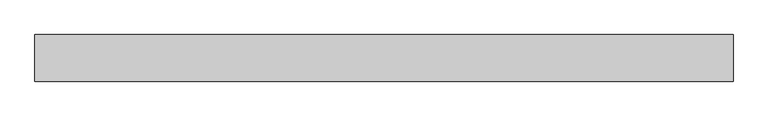
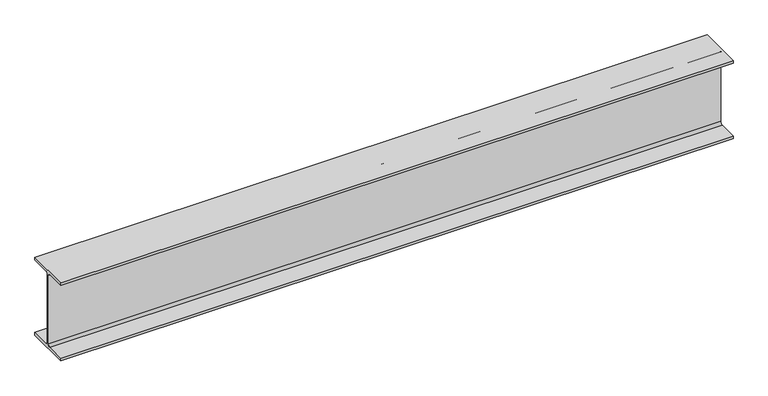
"""IFC4 building model written with IfcOpenShell, lengths in millimetres: beam geometry, Old_Steel Beam_H-KSD3502 : H_SB_ASB_H-350×175x7x11."""

import ifcopenshell
import ifcopenshell.guid

model = None  # the IFC model being written
_history = None  # IfcOwnerHistory: only IFC2X3 demands one
_inside = {}  # id of a spatial element -> (the spatial element, [elements in it])
_under = {}  # id of a project, library or spatial element -> (it, [spatial elements below it])
_declared = {}  # id of a project -> (the project, [libraries it declares])
_typed = {}  # id of a type object -> (the type object, [elements of that type])
_made_of = {}  # id of a material, layer set ... -> (it, [elements and type objects made of it])


def new_model(schema):
    """Start an empty IFC model of exactly this schema.

    Asked for "IFC4X3", IfcOpenShell would pick the latest addendum, in which some entities
    have other attributes; the version numbers below select the first issue.
    IFC2X3 requires an IfcOwnerHistory on every rooted entity: one is made here for all.
    """
    global model, _history
    if schema == "IFC4X3":
        model = ifcopenshell.file(schema_version=(4, 3, 0, 0))
    else:
        model = ifcopenshell.file(schema=schema)
    _inside.clear()
    _under.clear()
    _declared.clear()
    _typed.clear()
    _made_of.clear()
    _history = None
    if model.schema == "IFC2X3":
        org = make("IfcOrganization", Name="unknown")
        user = make(
            "IfcPersonAndOrganization",
            ThePerson=make("IfcPerson", FamilyName="unknown"),
            TheOrganization=org,
        )
        app = make(
            "IfcApplication",
            ApplicationDeveloper=org,
            Version="unknown",
            ApplicationFullName="unknown",
            ApplicationIdentifier="unknown",
        )
        _history = make(
            "IfcOwnerHistory",
            OwningUser=user,
            OwningApplication=app,
            ChangeAction="ADDED",
            CreationDate=0,
        )
    return model


def make(cls, **values):
    """One entity of the class cls with the attributes given. An attribute that is None is left unset."""
    return model.create_entity(
        cls, **{name: value for name, value in values.items() if value is not None}
    )


def rooted(cls, **values):
    """An entity with a GlobalId (a new one), such as an element, a storey or a relation."""
    return make(cls, GlobalId=ifcopenshell.guid.new(), OwnerHistory=_history, **values)


def si_unit(unit_type, name, prefix=None):
    """IfcSIUnit, for example si_unit("LENGTHUNIT", "METRE", prefix="MILLI")."""
    return make("IfcSIUnit", UnitType=unit_type, Prefix=prefix, Name=name)


def assignment(units):
    """IfcUnitAssignment: the units of a project."""
    return None if units is None else make("IfcUnitAssignment", Units=units)


def point(xyz):
    """IfcCartesianPoint."""
    return None if xyz is None else make("IfcCartesianPoint", Coordinates=xyz)


def direction(xyz):
    """IfcDirection."""
    return None if xyz is None else make("IfcDirection", DirectionRatios=xyz)


def frame(location, z_axis=None, x_axis=None):
    """IfcAxis2Placement3D, a coordinate frame: its origin and axes. An axis left out is left unset."""
    return make(
        "IfcAxis2Placement3D",
        Location=point(location),
        Axis=direction(z_axis),
        RefDirection=direction(x_axis),
    )


def frame_2d(location, x_axis=None):
    """IfcAxis2Placement2D, a coordinate frame in the plane: its origin and x axis."""
    return make(
        "IfcAxis2Placement2D", Location=point(location), RefDirection=direction(x_axis)
    )


def origin():
    """The frame at (0, 0, 0) with its axes left unset."""
    return frame((0.0, 0.0, 0.0))


def place(relative_to, where):
    """IfcLocalPlacement: puts the frame where relative to a parent placement (None: the world)."""
    return make(
        "IfcLocalPlacement", PlacementRelTo=relative_to, RelativePlacement=where
    )


def context(
    kind, dimensions, precision=None, world=None, true_north=None, identifier=None
):
    """IfcGeometricRepresentationContext, for example the 3D "Model" context."""
    return make(
        "IfcGeometricRepresentationContext",
        ContextIdentifier=identifier,
        ContextType=kind,
        CoordinateSpaceDimension=dimensions,
        Precision=precision,
        WorldCoordinateSystem=world,
        TrueNorth=true_north,
    )


def project(units=None, contexts=None):
    """IfcProject with its units and contexts."""
    return rooted(
        "IfcProject",
        Name="project",
        RepresentationContexts=contexts,
        UnitsInContext=assignment(units),
    )


def spatial(cls, under=None, at=None, **own):
    """A site, building, storey or space (cls), placed at a placement, below another one or the project."""
    s = rooted(cls, ObjectPlacement=at, **own)
    if under is not None:
        _under.setdefault(under.id(), (under, []))[1].append(s)
    return s


def polyline(points):
    """IfcPolyline through the points."""
    return make("IfcPolyline", Points=[point(p) for p in points])


def circle_curve(where, radius):
    """IfcCircle in the frame where."""
    return make("IfcCircle", Position=where, Radius=radius)


def trimmed(basis, trim1, trim2, sense, master):
    """IfcTrimmedCurve: the piece of a basis curve between two trims."""
    return make(
        "IfcTrimmedCurve",
        BasisCurve=basis,
        Trim1=trim1,
        Trim2=trim2,
        SenseAgreement=sense,
        MasterRepresentation=master,
    )


def segment(curve, same_sense, transition):
    """IfcCompositeCurveSegment."""
    return make(
        "IfcCompositeCurveSegment",
        Transition=transition,
        SameSense=same_sense,
        ParentCurve=curve,
    )


def composite_curve(segments, self_intersect=None):
    """IfcCompositeCurve: segments joined end to end."""
    return make("IfcCompositeCurve", Segments=segments, SelfIntersect=self_intersect)


def outline(outer, holes=None, kind="AREA"):
    """IfcArbitraryClosedProfileDef: a profile drawn as a closed curve; with holes, ...WithVoids."""
    if holes is None:
        return make("IfcArbitraryClosedProfileDef", ProfileType=kind, OuterCurve=outer)
    return make(
        "IfcArbitraryProfileDefWithVoids",
        ProfileType=kind,
        OuterCurve=outer,
        InnerCurves=holes,
    )


def extrude(swept, where, along, depth):
    """IfcExtrudedAreaSolid: the profile swept, set in the frame where, extruded along a direction by depth."""
    return make(
        "IfcExtrudedAreaSolid",
        SweptArea=swept,
        Position=where,
        ExtrudedDirection=direction(along),
        Depth=depth,
    )


def shape(context_of_items, identifier, shape_type, items):
    """IfcShapeRepresentation: the items that make up one representation, for example the "Body"."""
    return make(
        "IfcShapeRepresentation",
        ContextOfItems=context_of_items,
        RepresentationIdentifier=identifier,
        RepresentationType=shape_type,
        Items=items,
    )


def source(mapping_origin, context_of_items, identifier, shape_type, items):
    """IfcRepresentationMap: a shape defined once, which mapped items show again and again."""
    return make(
        "IfcRepresentationMap",
        MappingOrigin=mapping_origin,
        MappedRepresentation=shape(context_of_items, identifier, shape_type, items),
    )


def transform(
    local_origin,
    x_axis=None,
    y_axis=None,
    z_axis=None,
    scale=None,
    scale2=None,
    scale3=None,
    uniform=True,
):
    """IfcCartesianTransformationOperator3D, or its non-uniform kind. x_axis, y_axis, z_axis: its Axis1, 2, 3."""
    if uniform:
        return make(
            "IfcCartesianTransformationOperator3D",
            Axis1=direction(x_axis),
            Axis2=direction(y_axis),
            LocalOrigin=point(local_origin),
            Scale=scale,
            Axis3=direction(z_axis),
        )
    return make(
        "IfcCartesianTransformationOperator3DnonUniform",
        Axis1=direction(x_axis),
        Axis2=direction(y_axis),
        LocalOrigin=point(local_origin),
        Scale=scale,
        Axis3=direction(z_axis),
        Scale2=scale2,
        Scale3=scale3,
    )


def mapped(mapping_source, mapping_target):
    """IfcMappedItem: shows the shape of a source again, moved by a transform."""
    return make(
        "IfcMappedItem", MappingSource=mapping_source, MappingTarget=mapping_target
    )


def made_of(thing, what):
    """Note that an element or type object is made of a material, layer set ...; save() writes the relation."""
    if what is not None:
        _made_of.setdefault(what.id(), (what, []))[1].append(thing)
    return thing


def element(
    cls,
    number,
    at=None,
    inside=None,
    cuts=None,
    type_object=None,
    material=None,
    context=None,
    identifier="Body",
    shape_type=None,
    held_by="IfcProductDefinitionShape",
    body=None,
    shapes=None,
    **own,
):
    """One element of the class cls, such as IfcWall. Its Tag is "e" and its number.

    at: its placement. inside: the storey or other place that contains it. cuts: it is an
    opening in that element (IfcRelVoidsElement). A single representation is given by context,
    identifier, shape_type and body (its items); several are given by shapes. held_by: the class
    of the entity that holds the representations. save() writes the other relations.
    """
    e = rooted(cls, Tag="e%d" % number, ObjectPlacement=at, **own)
    if body is not None:
        shapes = [shape(context, identifier, shape_type, body)]
    if shapes is not None:
        e.Representation = make(held_by, Representations=shapes)
    if inside is not None:
        _inside.setdefault(inside.id(), (inside, []))[1].append(e)
    if cuts is not None:
        rooted(
            "IfcRelVoidsElement", RelatingBuildingElement=cuts, RelatedOpeningElement=e
        )
    if type_object is not None:
        _typed.setdefault(type_object.id(), (type_object, []))[1].append(e)
    return made_of(e, material)


def aggregate(whole, parts):
    """IfcRelAggregates: a whole, such as a stair, and the parts it consists of."""
    return rooted("IfcRelAggregates", RelatingObject=whole, RelatedObjects=parts)


def save(model, path):
    """Write the relations noted so far, then the file.

    IfcRelAggregates (storeys below a building ...), IfcRelContainedInSpatialStructure (elements
    in a storey), IfcRelDefinesByType, IfcRelAssociatesMaterial and IfcRelDeclares: one each for
    every whole, place, type object, material and project.
    """
    for whole, parts in _under.values():
        aggregate(whole, parts)
    for where, things in _inside.values():
        rooted(
            "IfcRelContainedInSpatialStructure",
            RelatedElements=things,
            RelatingStructure=where,
        )
    for kind, things in _typed.values():
        rooted("IfcRelDefinesByType", RelatedObjects=things, RelatingType=kind)
    for what, things in _made_of.values():
        rooted("IfcRelAssociatesMaterial", RelatedObjects=things, RelatingMaterial=what)
    for by, libraries in _declared.values():
        rooted("IfcRelDeclares", RelatingContext=by, RelatedDefinitions=libraries)
    model.write(path)


def beam_ab680fa0(model_context):
    return source(origin(), model_context, "Body", "SweptSolid", [
        extrude(outline(composite_curve([segment(polyline([(82.5, -141.5), (82.5, -151.7), (-82.5, -151.7), (-82.5, -141.5), (-11.9, -141.5)]), True, "CONTINUOUS"), segment(trimmed(circle_curve(frame_2d((-11.9, -132.6)), 8.9), [point((-11.9, -141.5))], [point((-3.0, -132.6))], True, "CARTESIAN"), True, "CONTINUOUS"), segment(polyline([(-3.0, -132.6), (-3.0, 132.6)]), True, "CONTINUOUS"), segment(trimmed(circle_curve(frame_2d((-11.9, 132.6)), 8.9), [point((-3.0, 132.6))], [point((-11.9, 141.5))], True, "CARTESIAN"), True, "CONTINUOUS"), segment(polyline([(-11.9, 141.5), (-82.5, 141.5), (-82.5, 151.7), (82.5, 151.7), (82.5, 141.5), (11.9, 141.5)]), True, "CONTINUOUS"), segment(trimmed(circle_curve(frame_2d((11.9, 132.6)), 8.9), [point((11.9, 141.5))], [point((3.0, 132.6))], True, "CARTESIAN"), True, "CONTINUOUS"), segment(polyline([(3.0, 132.6), (3.0, -132.6)]), True, "CONTINUOUS"), segment(trimmed(circle_curve(frame_2d((11.9, -132.6)), 8.9), [point((3.0, -132.6))], [point((11.9, -141.5))], True, "CARTESIAN"), True, "CONTINUOUS"), segment(polyline([(11.9, -141.5), (82.5, -141.5)]), True, "CONTINUOUS")], self_intersect=False)), frame((-1295.7739051, 0.0, 0.0), z_axis=(1.0, 0.0, 0.0), x_axis=(0.0, 1.0, 0.0)), (0.0, 0.0, 1.0), 2471.4118659),
    ])


if __name__ == "__main__":
    model = new_model("IFC4")
    model_context = context("Model", 3, world=origin())
    ifc_project = project(units=[si_unit("LENGTHUNIT", "METRE", prefix="MILLI")], contexts=[model_context])
    site = spatial("IfcSite", under=ifc_project)
    building = spatial("IfcBuilding", under=site)
    placement = place(None, origin())
    beam_shape = beam_ab680fa0(model_context)
    element("IfcBeam", 1, ObjectType="Old_Steel Beam_H-KSD3502 : H_SB_ASB_H-350×175x7x11", at=placement, inside=building, context=model_context, shape_type="MappedRepresentation", body=[
        mapped(beam_shape, transform((0.0, 0.0, 0.0), x_axis=(1.0, 0.0, 0.0), y_axis=(0.0, 1.0, 0.0), z_axis=(0.0, 0.0, 1.0))),
    ])
    save(model, "model.ifc")

# Revit data of these elements
# Type "Old_Steel Beam_H-KSD3502 : H_SB_ASB_H-350×175x7x11"
#   Width = 17.5 cm
#   Web Thickness = 0.7 cm
#   Web Fillet = 1.4 cm
#   Warping Constant = 282290.0 cm⁶
#   Torsional Moment of Inertia = 19.4042 cm⁴
#   Torsional Modulus = 1.0 cm³
#   Section Area = 63.14 cm²
#   Plastic Modulus weak axis = 174.0 cm³
#   Plastic Modulus strong axis = 868.0 cm³
#   Perimeter = 1.36 m²/m
#   Nominal Weight = 49.60 kgf/m
#   Moment of Inertia weak axis = 984.00 cm⁴
#   Moment of Inertia strong axis = 13600.00 cm⁴
#   Height = 35.0 cm
#   Flange Thickness = 1.1 cm
#   Elastic Modulus weak axis = 112.0 cm³
#   Elastic Modulus strong axis = 775.0 cm³
#   Centroid Vertical = 17.5 cm
#   Centroid Horizontal = 8.75 cm
#   Length [instance default] = 1.5240 m
#   Structural Material [instance default] = Steel, 45-345
#   Assembly Code = ""
# Element 1 (IfcBeam, "Old_Steel Beam_H-KSD3502 : H_SB_ASB_H-350×175x7x11")
#   Structural Material = none
# Materials
#   "Steel, 45-345": class "Metal", colour RGB 189 187 185, transparency 0, Description = "Steel 345 MPa", Cost = 0
